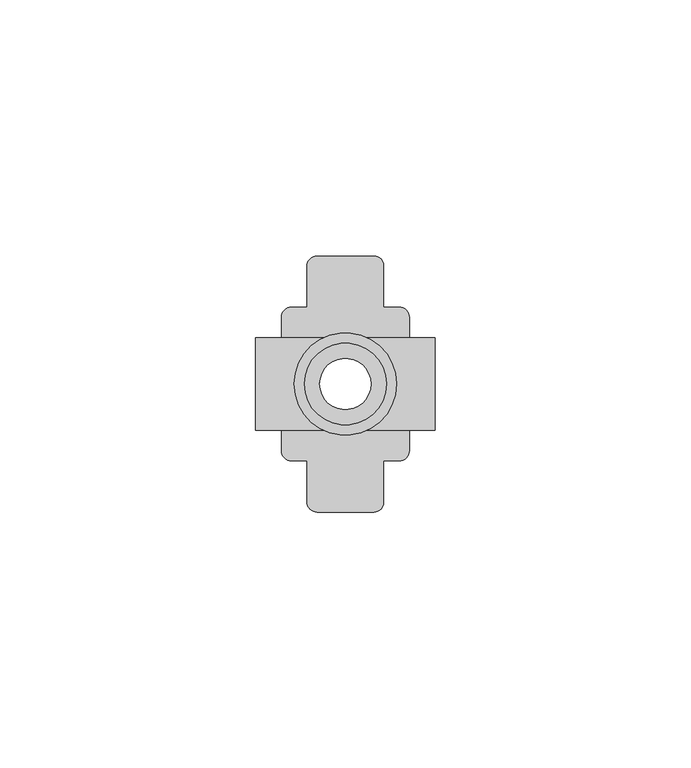
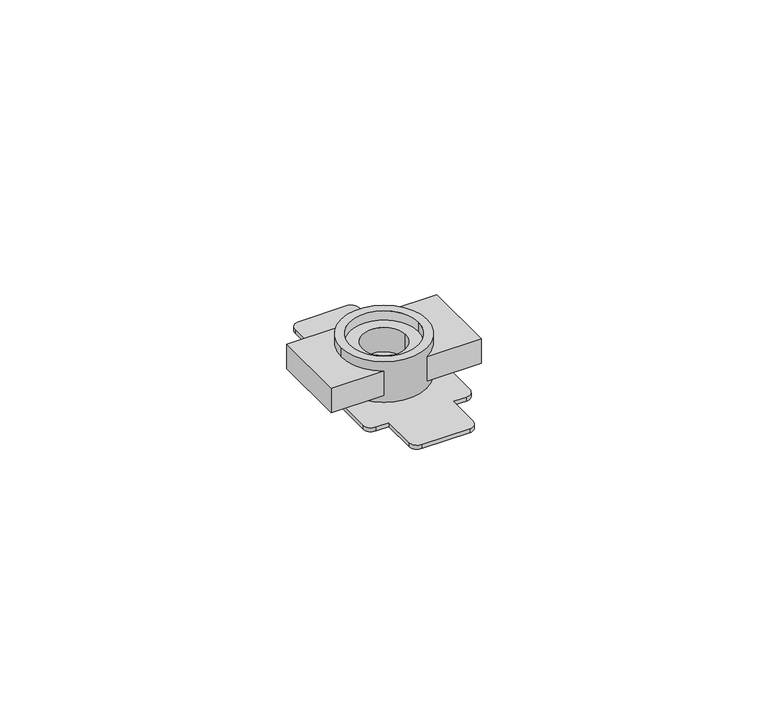
"""IFC4 building model written with IfcOpenShell, lengths in millimetres: proxy geometry, TN_Гайка быстрого монтажа потайная  : Гайка быстрого монтажа потайная 41 8F M10."""

from ifc_helpers import new_model, si_unit, point, frame, frame_2d, origin, origin_2d, place, context, project, spatial, polyline, circle_curve, trimmed, segment, composite_curve, outline, extrude, source, transform, mapped, element, save


def generic_models_cc5487ca(model_context):
    return source(origin(), model_context, "Body", "SweptSolid", [
        extrude(outline(composite_curve([segment(polyline([(-12.5, -13.0188504), (-12.5, 13.0188504)]), True, "CONTINUOUS"), segment(trimmed(circle_curve(frame_2d((-10.5188504, 13.0188504)), 1.9811496), [point((-12.5, 13.0188504))], [point((-10.5188504, 15.0))], False, "CARTESIAN"), True, "CONTINUOUS"), segment(polyline([(-10.5188504, 15.0), (-7.5, 15.0), (-7.5, 23.0)]), True, "CONTINUOUS"), segment(trimmed(circle_curve(frame_2d((-5.5, 23.0)), 2.0), [point((-7.5, 23.0))], [point((-5.5, 25.0))], False, "CARTESIAN"), True, "CONTINUOUS"), segment(polyline([(-5.5, 25.0), (5.5634262, 25.0)]), True, "CONTINUOUS"), segment(trimmed(circle_curve(frame_2d((5.5634262, 23.0634262)), 1.9365738), [point((5.5634262, 25.0))], [point((7.5, 23.0634262))], False, "CARTESIAN"), True, "CONTINUOUS"), segment(polyline([(7.5, 23.0634262), (7.5, 15.0), (10.5188504, 15.0)]), True, "CONTINUOUS"), segment(trimmed(circle_curve(frame_2d((10.5188504, 13.0188504)), 1.9811496), [point((10.5188504, 15.0))], [point((12.5, 13.0188504))], False, "CARTESIAN"), True, "CONTINUOUS"), segment(polyline([(12.5, 13.0188504), (12.5, -13.0188504)]), True, "CONTINUOUS"), segment(trimmed(circle_curve(frame_2d((10.5188504, -13.0188504)), 1.9811496), [point((12.5, -13.0188504))], [point((10.5188504, -15.0))], False, "CARTESIAN"), True, "CONTINUOUS"), segment(polyline([(10.5188504, -15.0), (7.5, -15.0), (7.5, -23.0634262)]), True, "CONTINUOUS"), segment(trimmed(circle_curve(frame_2d((5.5634262, -23.0634262)), 1.9365738), [point((7.5, -23.0634262))], [point((5.5634262, -25.0))], False, "CARTESIAN"), True, "CONTINUOUS"), segment(polyline([(5.5634262, -25.0), (-5.5, -25.0)]), True, "CONTINUOUS"), segment(trimmed(circle_curve(frame_2d((-5.5, -23.0)), 2.0), [point((-5.5, -25.0))], [point((-7.5, -23.0))], False, "CARTESIAN"), True, "CONTINUOUS"), segment(polyline([(-7.5, -23.0), (-7.5, -15.0), (-10.5188504, -15.0)]), True, "CONTINUOUS"), segment(trimmed(circle_curve(frame_2d((-10.5188504, -13.0188504)), 1.9811496), [point((-10.5188504, -15.0))], [point((-12.5, -13.0188504))], False, "CARTESIAN"), True, "CONTINUOUS")], self_intersect=False), holes=[composite_curve([segment(trimmed(circle_curve(origin_2d(), 5.0), [point((-5.0, 0.0))], [point((5.0, 0.0))], True, "CARTESIAN"), True, "CONTINUOUS"), segment(trimmed(circle_curve(origin_2d(), 5.0), [point((5.0, 0.0))], [point((-5.0, 0.0))], True, "CARTESIAN"), True, "CONTINUOUS")], self_intersect=False)]), frame((0.0, 0.0, -9.2966688), z_axis=(0.0, 0.0, 1.0), x_axis=(1.0, 0.0, 0.0)), (0.0, 0.0, 1.0), 1.0),
        extrude(outline(composite_curve([segment(trimmed(circle_curve(origin_2d(), 10.0), [point((-10.0, 0.0))], [point((10.0, 0.0))], False, "CARTESIAN"), True, "CONTINUOUS"), segment(trimmed(circle_curve(origin_2d(), 10.0), [point((10.0, 0.0))], [point((-10.0, 0.0))], False, "CARTESIAN"), True, "CONTINUOUS")], self_intersect=False), holes=[composite_curve([segment(trimmed(circle_curve(origin_2d(), 8.0), [point((-8.0, 0.0))], [point((8.0, 0.0))], True, "CARTESIAN"), True, "CONTINUOUS"), segment(trimmed(circle_curve(origin_2d(), 8.0), [point((8.0, 0.0))], [point((-8.0, 0.0))], True, "CARTESIAN"), True, "CONTINUOUS")], self_intersect=False)]), frame((0.0, 0.0, -8.2966688), z_axis=(0.0, 0.0, 1.0), x_axis=(1.0, 0.0, 0.0)), (0.0, 0.0, 1.0), 10.2966688),
        extrude(outline(polyline([(17.5, 9.0), (17.5, -9.0), (-17.5, -9.0), (-17.5, 9.0), (17.5, 9.0)]), holes=[composite_curve([segment(trimmed(circle_curve(origin_2d(), 5.0), [point((-5.0, 0.0))], [point((5.0, 0.0))], True, "CARTESIAN"), True, "CONTINUOUS"), segment(trimmed(circle_curve(origin_2d(), 5.0), [point((5.0, 0.0))], [point((-5.0, 0.0))], True, "CARTESIAN"), True, "CONTINUOUS")], self_intersect=False)]), frame((0.0, 0.0, -6.0), z_axis=(0.0, 0.0, 1.0), x_axis=(1.0, 0.0, 0.0)), (0.0, 0.0, 1.0), 6.0),
    ])


if __name__ == "__main__":
    model = new_model("IFC4")
    model_context = context("Model", 3, world=origin())
    ifc_project = project(units=[si_unit("LENGTHUNIT", "METRE", prefix="MILLI")], contexts=[model_context])
    site = spatial("IfcSite", under=ifc_project)
    building = spatial("IfcBuilding", under=site)
    placement = place(None, origin())
    generic_models_shape = generic_models_cc5487ca(model_context)
    element("IfcBuildingElementProxy", 1, Name="TN_Гайка быстрого монтажа потайная  : Гайка быстрого монтажа потайная 41 8F M10", ObjectType="TN_Гайка быстрого монтажа потайная  : Гайка быстрого монтажа потайная 41 8F M10", at=placement, inside=building, context=model_context, shape_type="MappedRepresentation", body=[
        mapped(generic_models_shape, transform((0.0, 0.0, 0.0), x_axis=(1.0, 0.0, 0.0), y_axis=(0.0, 1.0, 0.0), z_axis=(0.0, 0.0, 1.0))),
    ])
    save(model, "model.ifc")

# Revit data of these elements
# Type "TN_Гайка быстрого монтажа потайная  : Гайка быстрого монтажа потайная 41 8F M10"
#   Description = "Для надежного и быстрого закрепления заподлицо монтажных деталей, например, монтажных уголков в канавке тяжелого профиля. Сталь 6 / 8 мм; гальваническое покрытие цинком; полиамид."
#   Manufacturer = "ТехноНИКОЛЬ"
#   Model = "Комплектующие к опорам"
#   URL = "https://nav.tn.ru/knowledge-base/polimernye-membrany/opory-pod-oborudovanie-na-ploskoy-krovle/?sphrase_id=266812"
#   ADSK_Обозначение = "ТехноНИКОЛЬ"
#   ADSK_Наименование краткое = "41 8F M10"
#   ADSK_Наименование = "Гайка быстрого монтажа потайная 41 8F M10"
#   ADSK_Масса_Текст = ""
#   ADSK_Марка = "41 8F M10"
#   ADSK_Код изделия = "660823"
#   ADSK_Завод-изготовитель = "ТехноНИКОЛЬ"
#   ADSK_Единица измерения = "шт."
#   ADSK_Группирование = "Комплектующие к опорам"
#   ADSK_URL страницы изделия = "https://nav.tn.ru/knowledge-base/polimernye-membrany/opory-pod-oborudovanie-na-ploskoy-krovle/?sphrase_id=266812"
#   ADSK_URL документации изделия = ""
#   ADSK_Количество = 1
#   Метриал_Пластик = TN_Пластик_Красный
#   ADSK_Материал = TN_СтальГальванизированная_Серый
#   Default Elevation = 0
# Element 1 (IfcBuildingElementProxy, "TN_Гайка быстрого монтажа потайная  : Гайка быстрого монтажа потайная 41 8F M10")
#   Materials on its faces: "TN_Пластик_Красный", "TN_СтальГальванизированная_Серый"
# Materials
#   "TN_Пластик_Красный": class "Типовые", colour RGB 200 10 50, transparency 0, Cost = 0
#   "TN_СтальГальванизированная_Серый": class "Типовые", colour RGB 206 210 213, transparency 0, Cost = 0
